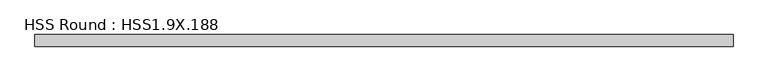
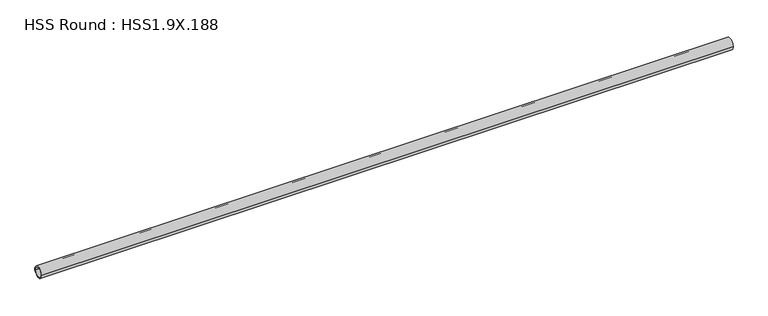
"""IFC4 building model written with IfcOpenShell, lengths in millimetres: member geometry, HSS Round : HSS1.9X.188."""

from ifc_helpers import new_model, si_unit, point, frame, origin, origin_2d, place, context, project, spatial, circle_curve, trimmed, segment, composite_curve, outline, extrude, source, transform, mapped, element, save


def hss_round_hss1_9x_188_89516c9e(model_context):
    return source(origin(), model_context, "Body", "SweptSolid", [
        extrude(outline(composite_curve([segment(trimmed(circle_curve(origin_2d(), 24.13), [point((-24.13, 0.0))], [point((24.13, 0.0))], False, "CARTESIAN"), True, "CONTINUOUS"), segment(trimmed(circle_curve(origin_2d(), 24.13), [point((24.13, 0.0))], [point((-24.13, 0.0))], False, "CARTESIAN"), True, "CONTINUOUS")], self_intersect=False), holes=[composite_curve([segment(trimmed(circle_curve(origin_2d(), 19.3548), [point((19.3548, 0.0))], [point((-19.3548, 0.0))], True, "CARTESIAN"), True, "CONTINUOUS"), segment(trimmed(circle_curve(origin_2d(), 19.3548), [point((-19.3548, 0.0))], [point((19.3548, 0.0))], True, "CARTESIAN"), True, "CONTINUOUS")], self_intersect=False)]), frame((-1489.0215058, 0.0, 0.0), z_axis=(1.0, 0.0, 0.0), x_axis=(0.0, 1.0, 0.0)), (0.0, 0.0, 1.0), 2904.873221),
    ])


if __name__ == "__main__":
    model = new_model("IFC4")
    model_context = context("Model", 3, world=origin())
    ifc_project = project(units=[si_unit("LENGTHUNIT", "METRE", prefix="MILLI")], contexts=[model_context])
    site = spatial("IfcSite", under=ifc_project)
    building = spatial("IfcBuilding", under=site)
    placement = place(None, origin())
    hss_round_hss1_9x_188_shape = hss_round_hss1_9x_188_89516c9e(model_context)
    element("IfcMember", 1, ObjectType="HSS Round : HSS1.9X.188", at=placement, inside=building, context=model_context, shape_type="MappedRepresentation", body=[
        mapped(hss_round_hss1_9x_188_shape, transform((0.0, 0.0, 0.0), x_axis=(1.0, 0.0, 0.0), y_axis=(0.0, 1.0, 0.0), z_axis=(0.0, 0.0, 1.0))),
    ])
    save(model, "model.ifc")

# Revit data of these elements
# Type "HSS Round : HSS1.9X.188"
#   Section Name Key = "HSSRound 1.900x0.188"
#   Assembly Code = "B10"
#   Wall Nominal Thickness = 0.188"
#   Wall Design Thickness = 0.174"
#   Torsional Moment of Inertia = 0.71 in⁴
#   Torsional Modulus = 0.747 in³
#   Section Area = 0.943 in²
#   Plastic Modulus weak axis = 0.52 in³
#   Plastic Modulus strong axis = 0.52 in³
#   Nominal Weight = 3.44 lbf/ft
#   Moment of Inertia weak axis = 0.355 in⁴
#   Moment of Inertia strong axis = 0.355 in⁴
#   Elastic Modulus weak axis = 0.374 in³
#   Elastic Modulus strong axis = 0.374 in³
#   Diameter = 1.900"
#   Centroid Vertical = 0.950"
#   Centroid Horizontal = 0.950"
#   Length [instance default] = 5' - 0"
#   Structural Material [instance default] = Steel ASTM A500, Grade B, Round
#   Warping Constant = (empty or 0)
#   Principal Axes Angle = 0
# Element 1 (IfcMember, "HSS Round : HSS1.9X.188")
#   Structural Material = Steel ASTM A992
#   Materials on its faces: "Steel ASTM A992"
# Materials
#   "Steel ASTM A500, Grade B, Round": class "Metal", colour RGB 199 199 199, transparency 0, Description = "Carbon steel", Cost = 0
#   "Steel ASTM A992": class "Metal", colour RGB 199 199 199, transparency 0, Description = "Structural steel 50ksi", Cost = 0
